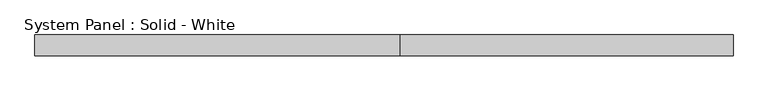
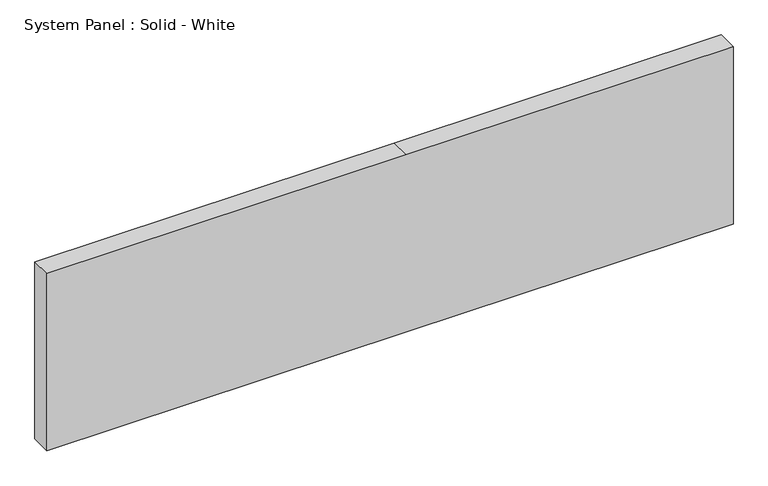
"""IFC4 building model written with IfcOpenShell, lengths in millimetres: plate geometry, System Panel : Solid - White."""

import ifcopenshell
import ifcopenshell.guid

model = None  # the IFC model being written
_history = None  # IfcOwnerHistory: only IFC2X3 demands one
_inside = {}  # id of a spatial element -> (the spatial element, [elements in it])
_under = {}  # id of a project, library or spatial element -> (it, [spatial elements below it])
_declared = {}  # id of a project -> (the project, [libraries it declares])
_typed = {}  # id of a type object -> (the type object, [elements of that type])
_made_of = {}  # id of a material, layer set ... -> (it, [elements and type objects made of it])


def new_model(schema):
    """Start an empty IFC model of exactly this schema.

    Asked for "IFC4X3", IfcOpenShell would pick the latest addendum, in which some entities
    have other attributes; the version numbers below select the first issue.
    IFC2X3 requires an IfcOwnerHistory on every rooted entity: one is made here for all.
    """
    global model, _history
    if schema == "IFC4X3":
        model = ifcopenshell.file(schema_version=(4, 3, 0, 0))
    else:
        model = ifcopenshell.file(schema=schema)
    _inside.clear()
    _under.clear()
    _declared.clear()
    _typed.clear()
    _made_of.clear()
    _history = None
    if model.schema == "IFC2X3":
        org = make("IfcOrganization", Name="unknown")
        user = make(
            "IfcPersonAndOrganization",
            ThePerson=make("IfcPerson", FamilyName="unknown"),
            TheOrganization=org,
        )
        app = make(
            "IfcApplication",
            ApplicationDeveloper=org,
            Version="unknown",
            ApplicationFullName="unknown",
            ApplicationIdentifier="unknown",
        )
        _history = make(
            "IfcOwnerHistory",
            OwningUser=user,
            OwningApplication=app,
            ChangeAction="ADDED",
            CreationDate=0,
        )
    return model


def make(cls, **values):
    """One entity of the class cls with the attributes given. An attribute that is None is left unset."""
    return model.create_entity(
        cls, **{name: value for name, value in values.items() if value is not None}
    )


def rooted(cls, **values):
    """An entity with a GlobalId (a new one), such as an element, a storey or a relation."""
    return make(cls, GlobalId=ifcopenshell.guid.new(), OwnerHistory=_history, **values)


def si_unit(unit_type, name, prefix=None):
    """IfcSIUnit, for example si_unit("LENGTHUNIT", "METRE", prefix="MILLI")."""
    return make("IfcSIUnit", UnitType=unit_type, Prefix=prefix, Name=name)


def assignment(units):
    """IfcUnitAssignment: the units of a project."""
    return None if units is None else make("IfcUnitAssignment", Units=units)


def point(xyz):
    """IfcCartesianPoint."""
    return None if xyz is None else make("IfcCartesianPoint", Coordinates=xyz)


def direction(xyz):
    """IfcDirection."""
    return None if xyz is None else make("IfcDirection", DirectionRatios=xyz)


def frame(location, z_axis=None, x_axis=None):
    """IfcAxis2Placement3D, a coordinate frame: its origin and axes. An axis left out is left unset."""
    return make(
        "IfcAxis2Placement3D",
        Location=point(location),
        Axis=direction(z_axis),
        RefDirection=direction(x_axis),
    )


def origin():
    """The frame at (0, 0, 0) with its axes left unset."""
    return frame((0.0, 0.0, 0.0))


def place(relative_to, where):
    """IfcLocalPlacement: puts the frame where relative to a parent placement (None: the world)."""
    return make(
        "IfcLocalPlacement", PlacementRelTo=relative_to, RelativePlacement=where
    )


def context(
    kind, dimensions, precision=None, world=None, true_north=None, identifier=None
):
    """IfcGeometricRepresentationContext, for example the 3D "Model" context."""
    return make(
        "IfcGeometricRepresentationContext",
        ContextIdentifier=identifier,
        ContextType=kind,
        CoordinateSpaceDimension=dimensions,
        Precision=precision,
        WorldCoordinateSystem=world,
        TrueNorth=true_north,
    )


def project(units=None, contexts=None):
    """IfcProject with its units and contexts."""
    return rooted(
        "IfcProject",
        Name="project",
        RepresentationContexts=contexts,
        UnitsInContext=assignment(units),
    )


def spatial(cls, under=None, at=None, **own):
    """A site, building, storey or space (cls), placed at a placement, below another one or the project."""
    s = rooted(cls, ObjectPlacement=at, **own)
    if under is not None:
        _under.setdefault(under.id(), (under, []))[1].append(s)
    return s


def polyline(points):
    """IfcPolyline through the points."""
    return make("IfcPolyline", Points=[point(p) for p in points])


def outline(outer, holes=None, kind="AREA"):
    """IfcArbitraryClosedProfileDef: a profile drawn as a closed curve; with holes, ...WithVoids."""
    if holes is None:
        return make("IfcArbitraryClosedProfileDef", ProfileType=kind, OuterCurve=outer)
    return make(
        "IfcArbitraryProfileDefWithVoids",
        ProfileType=kind,
        OuterCurve=outer,
        InnerCurves=holes,
    )


def extrude(swept, where, along, depth):
    """IfcExtrudedAreaSolid: the profile swept, set in the frame where, extruded along a direction by depth."""
    return make(
        "IfcExtrudedAreaSolid",
        SweptArea=swept,
        Position=where,
        ExtrudedDirection=direction(along),
        Depth=depth,
    )


def shape(context_of_items, identifier, shape_type, items):
    """IfcShapeRepresentation: the items that make up one representation, for example the "Body"."""
    return make(
        "IfcShapeRepresentation",
        ContextOfItems=context_of_items,
        RepresentationIdentifier=identifier,
        RepresentationType=shape_type,
        Items=items,
    )


def source(mapping_origin, context_of_items, identifier, shape_type, items):
    """IfcRepresentationMap: a shape defined once, which mapped items show again and again."""
    return make(
        "IfcRepresentationMap",
        MappingOrigin=mapping_origin,
        MappedRepresentation=shape(context_of_items, identifier, shape_type, items),
    )


def transform(
    local_origin,
    x_axis=None,
    y_axis=None,
    z_axis=None,
    scale=None,
    scale2=None,
    scale3=None,
    uniform=True,
):
    """IfcCartesianTransformationOperator3D, or its non-uniform kind. x_axis, y_axis, z_axis: its Axis1, 2, 3."""
    if uniform:
        return make(
            "IfcCartesianTransformationOperator3D",
            Axis1=direction(x_axis),
            Axis2=direction(y_axis),
            LocalOrigin=point(local_origin),
            Scale=scale,
            Axis3=direction(z_axis),
        )
    return make(
        "IfcCartesianTransformationOperator3DnonUniform",
        Axis1=direction(x_axis),
        Axis2=direction(y_axis),
        LocalOrigin=point(local_origin),
        Scale=scale,
        Axis3=direction(z_axis),
        Scale2=scale2,
        Scale3=scale3,
    )


def mapped(mapping_source, mapping_target):
    """IfcMappedItem: shows the shape of a source again, moved by a transform."""
    return make(
        "IfcMappedItem", MappingSource=mapping_source, MappingTarget=mapping_target
    )


def made_of(thing, what):
    """Note that an element or type object is made of a material, layer set ...; save() writes the relation."""
    if what is not None:
        _made_of.setdefault(what.id(), (what, []))[1].append(thing)
    return thing


def element(
    cls,
    number,
    at=None,
    inside=None,
    cuts=None,
    type_object=None,
    material=None,
    context=None,
    identifier="Body",
    shape_type=None,
    held_by="IfcProductDefinitionShape",
    body=None,
    shapes=None,
    **own,
):
    """One element of the class cls, such as IfcWall. Its Tag is "e" and its number.

    at: its placement. inside: the storey or other place that contains it. cuts: it is an
    opening in that element (IfcRelVoidsElement). A single representation is given by context,
    identifier, shape_type and body (its items); several are given by shapes. held_by: the class
    of the entity that holds the representations. save() writes the other relations.
    """
    e = rooted(cls, Tag="e%d" % number, ObjectPlacement=at, **own)
    if body is not None:
        shapes = [shape(context, identifier, shape_type, body)]
    if shapes is not None:
        e.Representation = make(held_by, Representations=shapes)
    if inside is not None:
        _inside.setdefault(inside.id(), (inside, []))[1].append(e)
    if cuts is not None:
        rooted(
            "IfcRelVoidsElement", RelatingBuildingElement=cuts, RelatedOpeningElement=e
        )
    if type_object is not None:
        _typed.setdefault(type_object.id(), (type_object, []))[1].append(e)
    return made_of(e, material)


def aggregate(whole, parts):
    """IfcRelAggregates: a whole, such as a stair, and the parts it consists of."""
    return rooted("IfcRelAggregates", RelatingObject=whole, RelatedObjects=parts)


def save(model, path):
    """Write the relations noted so far, then the file.

    IfcRelAggregates (storeys below a building ...), IfcRelContainedInSpatialStructure (elements
    in a storey), IfcRelDefinesByType, IfcRelAssociatesMaterial and IfcRelDeclares: one each for
    every whole, place, type object, material and project.
    """
    for whole, parts in _under.values():
        aggregate(whole, parts)
    for where, things in _inside.values():
        rooted(
            "IfcRelContainedInSpatialStructure",
            RelatedElements=things,
            RelatingStructure=where,
        )
    for kind, things in _typed.values():
        rooted("IfcRelDefinesByType", RelatedObjects=things, RelatingType=kind)
    for what, things in _made_of.values():
        rooted("IfcRelAssociatesMaterial", RelatedObjects=things, RelatingMaterial=what)
    for by, libraries in _declared.values():
        rooted("IfcRelDeclares", RelatingContext=by, RelatedDefinitions=libraries)
    model.write(path)


def system_panel_solid_white_3d2d69ba(model_context):
    return source(origin(), model_context, "Body", "SweptSolid", [
        extrude(outline(polyline([(0.0, -1057.7285714), (0.0, 49.8928571), (0.0, 1057.7285714), (577.85, 1057.7285714), (577.85, 49.8928571), (577.85, -1057.7285714), (0.0, -1057.7285714)])), frame((0.0, -19.05, 0.0), z_axis=(0.0, 1.0, 0.0), x_axis=(0.0, 0.0, 1.0)), (0.0, 0.0, 1.0), 63.5),
    ])


if __name__ == "__main__":
    model = new_model("IFC4")
    model_context = context("Model", 3, world=origin())
    ifc_project = project(units=[si_unit("LENGTHUNIT", "METRE", prefix="MILLI")], contexts=[model_context])
    site = spatial("IfcSite", under=ifc_project)
    building = spatial("IfcBuilding", under=site)
    placement = place(None, origin())
    system_panel_solid_white_shape = system_panel_solid_white_3d2d69ba(model_context)
    element("IfcPlate", 1, ObjectType="System Panel : Solid - White", at=placement, inside=building, context=model_context, shape_type="MappedRepresentation", body=[
        mapped(system_panel_solid_white_shape, transform((0.0, 0.0, 0.0), x_axis=(1.0, 0.0, 0.0), y_axis=(0.0, 1.0, 0.0), z_axis=(0.0, 0.0, 1.0))),
    ])
    save(model, "model.ifc")

# Revit data of these elements
# Project information
#   SR Document GUID = "e87cf156-1ea9-4512-a4ef-a5481400b45a"
# Element 1 (IfcPlate, "System Panel : Solid - White")
#   Materials on its faces: "White Panel"
# Materials
#   "White Panel": class "Unassigned", colour RGB 255 255 255, transparency 0
